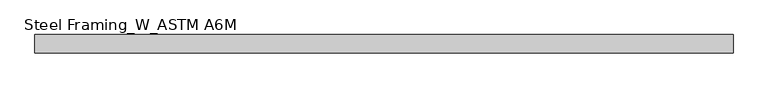
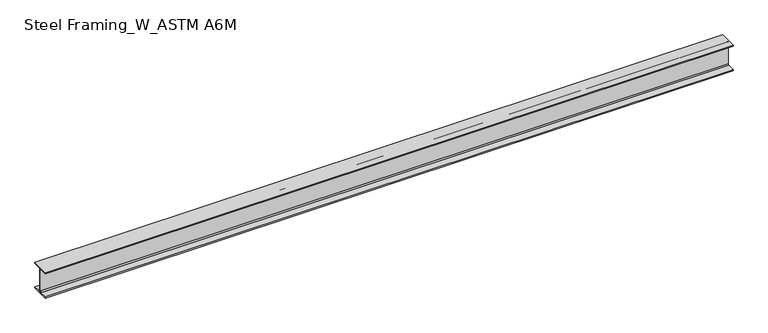
"""IFC4 building model written with IfcOpenShell, lengths in millimetres: beam geometry, Steel Framing_W_ASTM A6M : H_SB_AR_S02_W310x60_B5."""

from ifc_helpers import new_model, si_unit, point, frame, frame_2d, origin, place, context, project, spatial, polyline, circle_curve, trimmed, segment, composite_curve, outline, extrude, source, transform, mapped, element, save


def steel_framing_w_astm_a6m_97b597d5(model_context):
    return source(origin(), model_context, "Body", "SweptSolid", [
        extrude(outline(composite_curve([segment(polyline([(101.5, -137.9), (101.5, -151.0), (-101.5, -151.0), (-101.5, -137.9), (-16.545, -137.9)]), True, "CONTINUOUS"), segment(trimmed(circle_curve(frame_2d((-16.545, -125.1)), 12.8), [point((-16.545, -137.9))], [point((-3.745, -125.1))], True, "CARTESIAN"), True, "CONTINUOUS"), segment(polyline([(-3.745, -125.1), (-3.745, 125.1)]), True, "CONTINUOUS"), segment(trimmed(circle_curve(frame_2d((-16.545, 125.1)), 12.8), [point((-3.745, 125.1))], [point((-16.545, 137.9))], True, "CARTESIAN"), True, "CONTINUOUS"), segment(polyline([(-16.545, 137.9), (-101.5, 137.9), (-101.5, 151.0), (101.5, 151.0), (101.5, 137.9), (16.545, 137.9)]), True, "CONTINUOUS"), segment(trimmed(circle_curve(frame_2d((16.545, 125.1)), 12.8), [point((16.545, 137.9))], [point((3.745, 125.1))], True, "CARTESIAN"), True, "CONTINUOUS"), segment(polyline([(3.745, 125.1), (3.745, -125.1)]), True, "CONTINUOUS"), segment(trimmed(circle_curve(frame_2d((16.545, -125.1)), 12.8), [point((3.745, -125.1))], [point((16.545, -137.9))], True, "CARTESIAN"), True, "CONTINUOUS"), segment(polyline([(16.545, -137.9), (101.5, -137.9)]), True, "CONTINUOUS")], self_intersect=False)), frame((-3884.3, 0.0, 0.0), z_axis=(1.0, 0.0, 0.0), x_axis=(0.0, 1.0, 0.0)), (0.0, 0.0, 1.0), 7698.8),
    ])


if __name__ == "__main__":
    model = new_model("IFC4")
    model_context = context("Model", 3, world=origin())
    ifc_project = project(units=[si_unit("LENGTHUNIT", "METRE", prefix="MILLI")], contexts=[model_context])
    site = spatial("IfcSite", under=ifc_project)
    building = spatial("IfcBuilding", under=site)
    placement = place(None, origin())
    steel_framing_w_astm_a6m_shape = steel_framing_w_astm_a6m_97b597d5(model_context)
    element("IfcBeam", 1, ObjectType="Steel Framing_W_ASTM A6M : H_SB_AR_S02_W310x60_B5", at=placement, inside=building, context=model_context, shape_type="MappedRepresentation", body=[
        mapped(steel_framing_w_astm_a6m_shape, transform((0.0, 0.0, 0.0), x_axis=(1.0, 0.0, 0.0), y_axis=(0.0, 1.0, 0.0), z_axis=(0.0, 0.0, 1.0))),
    ])
    save(model, "model.ifc")

# Revit data of these elements
# Type "Steel Framing_W_ASTM A6M : H_SB_AR_S02_W310x60_B5"
#   Type Mark = "B5"
#   Section Name Key = "W12x40"
#   Width = 20.3 cm
#   Web Thickness = 0.749 cm
#   Web Fillet = 1.28 cm
#   Warping Constant = 387000.0 cm⁶
#   Torsional Moment of Inertia = 37.70 cm⁴
#   Section Area = 75.5 cm²
#   Plastic Modulus weak axis = 275.0 cm³
#   Plastic Modulus strong axis = 934.0 cm³
#   Perimeter = 1.38 m²/m
#   Nominal Weight = 60.00 kgf/m
#   Moment of Inertia weak axis = 1840.00 cm⁴
#   Moment of Inertia strong axis = 12800.00 cm⁴
#   Height = 30.2 cm
#   Flange Thickness = 1.31 cm
#   Elastic Modulus weak axis = 180.0 cm³
#   Elastic Modulus strong axis = 844.0 cm³
#   Centroid Vertical = 15.1 cm
#   Centroid Horizontal = 10.15 cm
#   Length [instance default] = 1500 mm
#   Structural Material [instance default] = Steel, 45-345
#   Bolt Spacing = 0
#   Assembly Code = ""
# Element 1 (IfcBeam, "Steel Framing_W_ASTM A6M : H_SB_AR_S02_W310x60_B5")
#   Materials on its faces: "Steel, 45-345"
# Materials
#   "Steel, 45-345": class "Metal", colour RGB 189 187 185, transparency 0, Description = "Steel 345 MPa", Cost = 0
